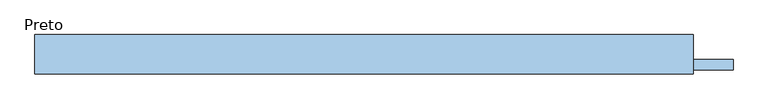
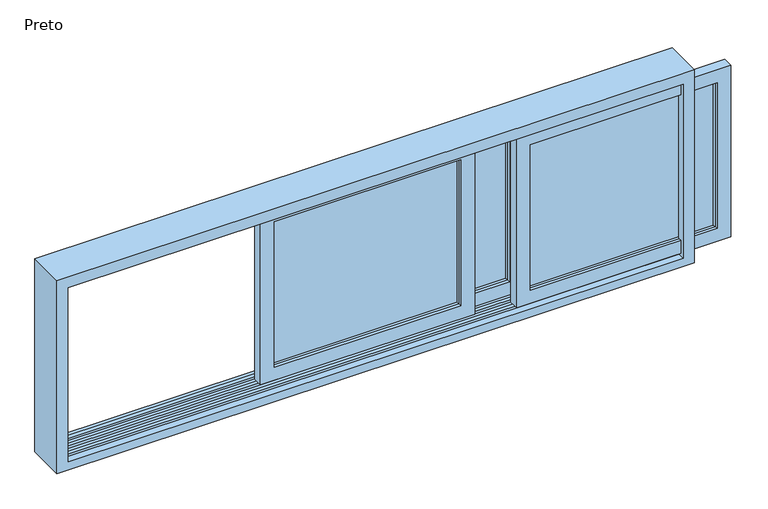
"""IFC4 building model written with IfcOpenShell, lengths in millimetres: window geometry, Blks_Cons Weiku_Janela de Correr 03 Folhas : Preto."""

from ifc_helpers import new_model, si_unit, frame, origin, place, context, project, spatial, polyline, outline, extrude, faceted_brep, source, transform, mapped, element, save


def preto_66575e38(model_context):
    return source(origin(), model_context, "Body", "SolidModel", [
        faceted_brep([(-152.0, 47.0, 898.0), (-152.0, 42.0, 898.0), (-152.0, 42.0, 1502.0), (-152.0, 47.0, 1502.0), (-147.0, 42.0, 903.0), (-147.0, 42.0, 1497.0), (580.0, 42.0, 1502.0), (580.0, 47.0, 1502.0), (575.0, 42.0, 1497.0), (580.0, 42.0, 898.0), (580.0, 47.0, 898.0), (575.0, 42.0, 903.0)], [[[0, 1, 2, 3]], [[4, 0, 3, 5]], [[3, 2, 6, 7]], [[5, 3, 7, 8]], [[7, 6, 9, 10]], [[8, 7, 10, 11]], [[1, 9, 6, 2], [5, 8, 11, 4]], [[10, 9, 1, 0]], [[11, 10, 0, 4]]]),
        faceted_brep([(580.0, 33.0, 898.0), (580.0, 38.0, 898.0), (580.0, 38.0, 1502.0), (580.0, 33.0, 1502.0), (-152.0, 38.0, 1502.0), (-152.0, 33.0, 1502.0), (-152.0, 38.0, 898.0), (-152.0, 33.0, 898.0), (575.0, 38.0, 1497.0), (-147.0, 38.0, 1497.0), (-147.0, 38.0, 903.0), (575.0, 38.0, 903.0)], [[[0, 1, 2, 3]], [[3, 2, 4, 5]], [[5, 4, 6, 7]], [[1, 6, 4, 2], [8, 9, 10, 11]], [[7, 6, 1, 0]], [[11, 0, 3, 8]], [[8, 3, 5, 9]], [[9, 5, 7, 10]], [[10, 7, 0, 11]]]),
        extrude(outline(polyline([(580.0, 38.0), (-152.0, 38.0), (-152.0, 42.0), (580.0, 42.0), (580.0, 38.0)])), frame((0.0, 0.0, 898.0), z_axis=(0.0, 0.0, 1.0), x_axis=(1.0, 0.0, 0.0)), (0.0, 0.0, 1.0), 604.0),
        extrude(outline(polyline([(844.0, 634.0), (1556.0, 634.0), (1556.0, -206.0), (844.0, -206.0), (844.0, 634.0)]), holes=[polyline([(1502.0, -152.0), (1502.0, 580.0), (898.0, 580.0), (898.0, -152.0), (1502.0, -152.0)])]), frame((0.0, 20.0, 0.0), z_axis=(0.0, 1.0, 0.0), x_axis=(0.0, 0.0, 1.0)), (0.0, 0.0, 1.0), 40.0),
        faceted_brep([(-366.0, 7.0, 898.0), (-366.0, 2.0, 898.0), (-366.0, 2.0, 1502.0), (-366.0, 7.0, 1502.0), (-361.0, 2.0, 903.0), (-361.0, 2.0, 1497.0), (366.0, 2.0, 1502.0), (366.0, 7.0, 1502.0), (361.0, 2.0, 1497.0), (366.0, 2.0, 898.0), (366.0, 7.0, 898.0), (361.0, 2.0, 903.0)], [[[0, 1, 2, 3]], [[4, 0, 3, 5]], [[3, 2, 6, 7]], [[5, 3, 7, 8]], [[7, 6, 9, 10]], [[8, 7, 10, 11]], [[1, 9, 6, 2], [5, 8, 11, 4]], [[10, 9, 1, 0]], [[11, 10, 0, 4]]]),
        faceted_brep([(366.0, -7.0, 898.0), (366.0, -2.0, 898.0), (366.0, -2.0, 1502.0), (366.0, -7.0, 1502.0), (-366.0, -2.0, 1502.0), (-366.0, -7.0, 1502.0), (-366.0, -2.0, 898.0), (-366.0, -7.0, 898.0), (361.0, -2.0, 1497.0), (-361.0, -2.0, 1497.0), (-361.0, -2.0, 903.0), (361.0, -2.0, 903.0)], [[[0, 1, 2, 3]], [[3, 2, 4, 5]], [[5, 4, 6, 7]], [[1, 6, 4, 2], [8, 9, 10, 11]], [[7, 6, 1, 0]], [[11, 0, 3, 8]], [[8, 3, 5, 9]], [[9, 5, 7, 10]], [[10, 7, 0, 11]]]),
        extrude(outline(polyline([(366.0, -2.0), (-366.0, -2.0), (-366.0, 2.0), (366.0, 2.0), (366.0, -2.0)])), frame((0.0, 0.0, 898.0), z_axis=(0.0, 0.0, 1.0), x_axis=(1.0, 0.0, 0.0)), (0.0, 0.0, 1.0), 604.0),
        extrude(outline(polyline([(844.0, 420.0), (1556.0, 420.0), (1556.0, -420.0), (844.0, -420.0), (844.0, 420.0)]), holes=[polyline([(1502.0, -366.0), (1502.0, 366.0), (898.0, 366.0), (898.0, -366.0), (1502.0, -366.0)])]), frame((0.0, -20.0, 0.0), z_axis=(0.0, 1.0, 0.0), x_axis=(0.0, 0.0, 1.0)), (0.0, 0.0, 1.0), 40.0),
        faceted_brep([(616.0, -33.0, 898.0), (616.0, -38.0, 898.0), (616.0, -38.0, 1502.0), (616.0, -33.0, 1502.0), (621.0, -38.0, 903.0), (621.0, -38.0, 1497.0), (1348.0, -38.0, 1502.0), (1348.0, -33.0, 1502.0), (1343.0, -38.0, 1497.0), (1348.0, -38.0, 898.0), (1348.0, -33.0, 898.0), (1343.0, -38.0, 903.0)], [[[0, 1, 2, 3]], [[4, 0, 3, 5]], [[3, 2, 6, 7]], [[5, 3, 7, 8]], [[7, 6, 9, 10]], [[8, 7, 10, 11]], [[1, 9, 6, 2], [5, 8, 11, 4]], [[10, 9, 1, 0]], [[11, 10, 0, 4]]]),
        faceted_brep([(1348.0, -47.0, 898.0), (1348.0, -42.0, 898.0), (1348.0, -42.0, 1502.0), (1348.0, -47.0, 1502.0), (616.0, -42.0, 1502.0), (616.0, -47.0, 1502.0), (616.0, -42.0, 898.0), (616.0, -47.0, 898.0), (1343.0, -42.0, 1497.0), (621.0, -42.0, 1497.0), (621.0, -42.0, 903.0), (1343.0, -42.0, 903.0)], [[[0, 1, 2, 3]], [[3, 2, 4, 5]], [[5, 4, 6, 7]], [[1, 6, 4, 2], [8, 9, 10, 11]], [[7, 6, 1, 0]], [[11, 0, 3, 8]], [[8, 3, 5, 9]], [[9, 5, 7, 10]], [[10, 7, 0, 11]]]),
        extrude(outline(polyline([(1348.0, -42.0), (616.0, -42.0), (616.0, -38.0), (1348.0, -38.0), (1348.0, -42.0)])), frame((0.0, 0.0, 898.0), z_axis=(0.0, 0.0, 1.0), x_axis=(1.0, 0.0, 0.0)), (0.0, 0.0, 1.0), 604.0),
        extrude(outline(polyline([(844.0, 1402.0), (1556.0, 1402.0), (1556.0, 562.0), (844.0, 562.0), (844.0, 1402.0)]), holes=[polyline([(1502.0, 616.0), (1502.0, 1348.0), (898.0, 1348.0), (898.0, 616.0), (1502.0, 616.0)])]), frame((0.0, -60.0, 0.0), z_axis=(0.0, 1.0, 0.0), x_axis=(0.0, 0.0, 1.0)), (0.0, 0.0, 1.0), 40.0),
        faceted_brep([(-1206.0, -33.0, 844.0), (-1206.0, -47.0, 844.0), (1206.0, -47.0, 844.0), (1206.0, -33.0, 844.0), (-1206.0, 7.0, 844.0), (-1206.0, -7.0, 844.0), (1206.0, -7.0, 844.0), (1206.0, 7.0, 844.0), (-1206.0, 47.0, 844.0), (-1206.0, 33.0, 844.0), (1206.0, 33.0, 844.0), (1206.0, 47.0, 844.0), (-1206.0, -33.0, 834.0), (-1206.0, -7.0, 834.0), (-1206.0, 7.0, 834.0), (-1206.0, 33.0, 834.0), (-1206.0, 47.0, 834.0), (-1206.0, 75.0, 834.0), (-1206.0, 75.0, 1556.0), (-1206.0, 60.0, 1556.0), (-1206.0, 60.0, 1566.0), (-1206.0, 42.0, 1566.0), (-1206.0, 42.0, 1556.0), (-1206.0, 28.0, 1556.0), (-1206.0, 28.0, 1566.0), (-1206.0, 2.0, 1566.0), (-1206.0, 2.0, 1556.0), (-1206.0, -12.0, 1556.0), (-1206.0, -12.0, 1566.0), (-1206.0, -38.0, 1566.0), (-1206.0, -38.0, 1556.0), (-1206.0, -52.0, 1556.0), (-1206.0, -52.0, 1566.0), (-1206.0, -60.0, 1566.0), (-1206.0, -60.0, 1556.0), (-1206.0, -75.0, 1556.0), (-1206.0, -75.0, 834.0), (-1206.0, -47.0, 834.0), (1206.0, -47.0, 834.0), (1206.0, -12.0, 1556.0), (1206.0, 2.0, 1556.0), (1206.0, 2.0, 1566.0), (1206.0, 28.0, 1566.0), (1206.0, 28.0, 1556.0), (1206.0, 42.0, 1556.0), (1206.0, 42.0, 1566.0), (1206.0, 60.0, 1566.0), (1206.0, 60.0, 1556.0), (1206.0, 75.0, 1556.0), (1206.0, 75.0, 834.0), (1206.0, 47.0, 834.0), (1206.0, 33.0, 834.0), (1206.0, 7.0, 834.0), (1206.0, -7.0, 834.0), (1206.0, -33.0, 834.0), (1206.0, -75.0, 834.0), (1206.0, -75.0, 1556.0), (1206.0, -60.0, 1556.0), (1206.0, -60.0, 1566.0), (1206.0, -52.0, 1566.0), (1206.0, -52.0, 1556.0), (1206.0, -38.0, 1556.0), (1206.0, -38.0, 1566.0), (1206.0, -12.0, 1566.0), (1250.0, -75.0, 800.0), (1250.0, 75.0, 800.0), (1250.0, 75.0, 1600.0), (1250.0, -75.0, 1600.0), (-1250.0, -75.0, 800.0), (-1250.0, 75.0, 800.0), (-1250.0, -75.0, 1600.0), (-1250.0, 75.0, 1600.0)], [[[0, 1, 2, 3]], [[4, 5, 6, 7]], [[8, 9, 10, 11]], [[1, 0, 12, 13, 5, 4, 14, 15, 9, 8, 16, 17, 18, 19, 20, 21, 22, 23, 24, 25, 26, 27, 28, 29, 30, 31, 32, 33, 34, 35, 36, 37]], [[38, 2, 1, 37]], [[39, 40, 41, 42, 43, 44, 45, 46, 47, 48, 49, 50, 11, 10, 51, 52, 7, 6, 53, 54, 3, 2, 38, 55, 56, 57, 58, 59, 60, 61, 62, 63]], [[3, 54, 12, 0]], [[53, 6, 5, 13]], [[7, 52, 14, 4]], [[51, 10, 9, 15]], [[11, 50, 16, 8]], [[64, 65, 66, 67]], [[65, 64, 68, 69]], [[68, 64, 67, 70], [36, 35, 56, 55]], [[69, 68, 70, 71]], [[65, 69, 71, 66], [49, 48, 18, 17]], [[54, 53, 13, 12]], [[52, 51, 15, 14]], [[50, 49, 17, 16]], [[55, 38, 37, 36]], [[23, 22, 44, 43]], [[27, 26, 40, 39]], [[31, 30, 61, 60]], [[18, 48, 47, 19]], [[56, 35, 34, 57]], [[71, 70, 67, 66]], [[43, 42, 24, 23]], [[42, 41, 25, 24]], [[41, 40, 26, 25]], [[39, 63, 28, 27]], [[63, 62, 29, 28]], [[62, 61, 30, 29]], [[60, 59, 32, 31]], [[59, 58, 33, 32]], [[33, 58, 57, 34]], [[46, 20, 19, 47]], [[46, 45, 21, 20]], [[45, 44, 22, 21]]]),
    ])


if __name__ == "__main__":
    model = new_model("IFC4")
    model_context = context("Model", 3, world=origin())
    ifc_project = project(units=[si_unit("LENGTHUNIT", "METRE", prefix="MILLI")], contexts=[model_context])
    site = spatial("IfcSite", under=ifc_project)
    building = spatial("IfcBuilding", under=site)
    placement = place(None, origin())
    preto_shape = preto_66575e38(model_context)
    element("IfcWindow", 1, ObjectType="Blks_Cons Weiku_Janela de Correr 03 Folhas : Preto", at=placement, inside=building, context=model_context, shape_type="MappedRepresentation", body=[
        mapped(preto_shape, transform((0.0, 0.0, 0.0), x_axis=(1.0, 0.0, 0.0), y_axis=(0.0, 1.0, 0.0), z_axis=(0.0, 0.0, 1.0))),
    ])
    save(model, "model.ifc")

# Revit data of these elements
# Type "Blks_Cons Weiku_Janela de Correr 03 Folhas : Preto"
#   Type Mark = "J23"
#   Type Comments = "Janela de Correr 03 Folhas"
#   Manufacturer = "Weiku"
#   Created By / Criado Por / Creado por = "Blocks"
#   Author URL = "https://BlocksRvt.com/"
#   Author Contact = "info@blocksrvt.com"
#   Assembly Code = "Cons"
#   b [instance default] = 912 mm
#   a [instance default] = 1036 mm
#   Width [instance default] = 3000 mm
#   Rough Width [instance default] = 3088 mm
#   Rough Height [instance default] = 1000 mm
#   Height [instance default] = 912 mm
#   Espessura Folha [instance default] = 40 mm
#   Abertura Folha Interna [instance default] = 75 mm
#   Abertura Folha Externa [instance default] = 1964 mm
#   Abertura Folha Central [instance default] = 982 mm
#   Vidro = .vidro_growarq
#   Vedação = Blks - Rubber - Black
#   Janela = Blks - Plastic - Black - Glazed
#   Wall Closure = (empty or 0)
# Element 1 (IfcWindow, "Blks_Cons Weiku_Janela de Correr 03 Folhas : Preto")
#   b = 712 mm
#   a = 840 mm
#   Width = 2412 mm
#   Rough Width = 2500 mm
#   Rough Height = 800 mm
#   Height = 712 mm
#   Abertura Folha Interna = 1000 mm
#   Abertura Folha Externa = 2200 mm
#   Abertura Folha Central = 900 mm
#   Materials on its faces: "Blks - Plastic - Black - Glazed", "Blks - Rubber - Black", ".vidro_growarq"
# Materials
#   ".vidro_growarq": class "Vidro", colour RGB 200 215 215, transparency 0.6, Description = "Vidroverde", Cost = 0
#   "Blks - Rubber - Black": class "Paint/Coating", colour RGB 38 38 38, transparency 0, Cost = 0
#   "Blks - Plastic - Black - Glazed": class "Plastic", colour RGB 25 25 25, transparency 0, Cost = 0
